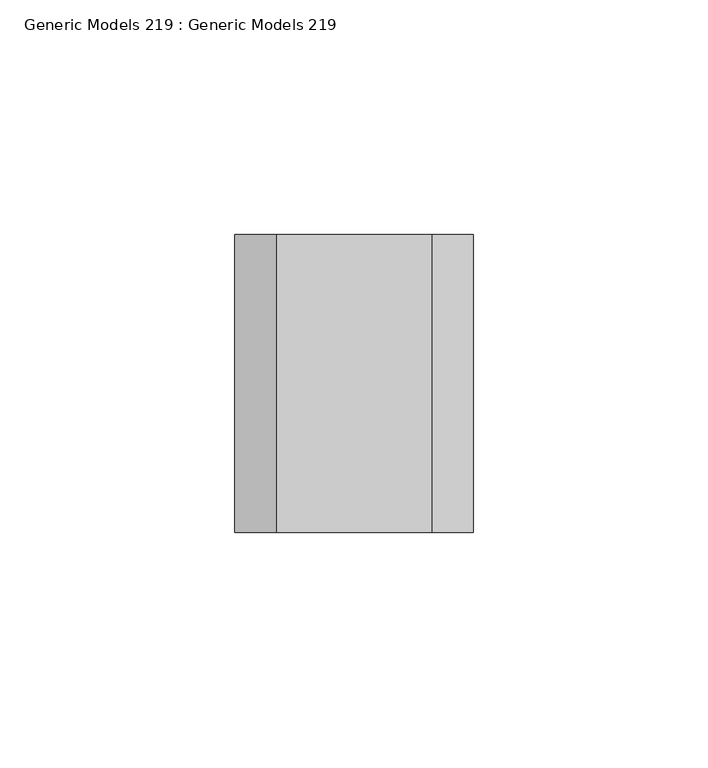
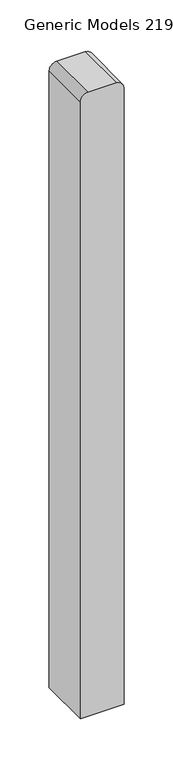
"""IFC4 building model written with IfcOpenShell, lengths in millimetres: proxy geometry, Generic Models 219 : Generic Models 219."""

import ifcopenshell
import ifcopenshell.guid

model = None  # the IFC model being written
_history = None  # IfcOwnerHistory: only IFC2X3 demands one
_inside = {}  # id of a spatial element -> (the spatial element, [elements in it])
_under = {}  # id of a project, library or spatial element -> (it, [spatial elements below it])
_declared = {}  # id of a project -> (the project, [libraries it declares])
_typed = {}  # id of a type object -> (the type object, [elements of that type])
_made_of = {}  # id of a material, layer set ... -> (it, [elements and type objects made of it])


def new_model(schema):
    """Start an empty IFC model of exactly this schema.

    Asked for "IFC4X3", IfcOpenShell would pick the latest addendum, in which some entities
    have other attributes; the version numbers below select the first issue.
    IFC2X3 requires an IfcOwnerHistory on every rooted entity: one is made here for all.
    """
    global model, _history
    if schema == "IFC4X3":
        model = ifcopenshell.file(schema_version=(4, 3, 0, 0))
    else:
        model = ifcopenshell.file(schema=schema)
    _inside.clear()
    _under.clear()
    _declared.clear()
    _typed.clear()
    _made_of.clear()
    _history = None
    if model.schema == "IFC2X3":
        org = make("IfcOrganization", Name="unknown")
        user = make(
            "IfcPersonAndOrganization",
            ThePerson=make("IfcPerson", FamilyName="unknown"),
            TheOrganization=org,
        )
        app = make(
            "IfcApplication",
            ApplicationDeveloper=org,
            Version="unknown",
            ApplicationFullName="unknown",
            ApplicationIdentifier="unknown",
        )
        _history = make(
            "IfcOwnerHistory",
            OwningUser=user,
            OwningApplication=app,
            ChangeAction="ADDED",
            CreationDate=0,
        )
    return model


def make(cls, **values):
    """One entity of the class cls with the attributes given. An attribute that is None is left unset."""
    return model.create_entity(
        cls, **{name: value for name, value in values.items() if value is not None}
    )


def rooted(cls, **values):
    """An entity with a GlobalId (a new one), such as an element, a storey or a relation."""
    return make(cls, GlobalId=ifcopenshell.guid.new(), OwnerHistory=_history, **values)


def si_unit(unit_type, name, prefix=None):
    """IfcSIUnit, for example si_unit("LENGTHUNIT", "METRE", prefix="MILLI")."""
    return make("IfcSIUnit", UnitType=unit_type, Prefix=prefix, Name=name)


def assignment(units):
    """IfcUnitAssignment: the units of a project."""
    return None if units is None else make("IfcUnitAssignment", Units=units)


def point(xyz):
    """IfcCartesianPoint."""
    return None if xyz is None else make("IfcCartesianPoint", Coordinates=xyz)


def direction(xyz):
    """IfcDirection."""
    return None if xyz is None else make("IfcDirection", DirectionRatios=xyz)


def frame(location, z_axis=None, x_axis=None):
    """IfcAxis2Placement3D, a coordinate frame: its origin and axes. An axis left out is left unset."""
    return make(
        "IfcAxis2Placement3D",
        Location=point(location),
        Axis=direction(z_axis),
        RefDirection=direction(x_axis),
    )


def frame_2d(location, x_axis=None):
    """IfcAxis2Placement2D, a coordinate frame in the plane: its origin and x axis."""
    return make(
        "IfcAxis2Placement2D", Location=point(location), RefDirection=direction(x_axis)
    )


def origin():
    """The frame at (0, 0, 0) with its axes left unset."""
    return frame((0.0, 0.0, 0.0))


def place(relative_to, where):
    """IfcLocalPlacement: puts the frame where relative to a parent placement (None: the world)."""
    return make(
        "IfcLocalPlacement", PlacementRelTo=relative_to, RelativePlacement=where
    )


def context(
    kind, dimensions, precision=None, world=None, true_north=None, identifier=None
):
    """IfcGeometricRepresentationContext, for example the 3D "Model" context."""
    return make(
        "IfcGeometricRepresentationContext",
        ContextIdentifier=identifier,
        ContextType=kind,
        CoordinateSpaceDimension=dimensions,
        Precision=precision,
        WorldCoordinateSystem=world,
        TrueNorth=true_north,
    )


def project(units=None, contexts=None):
    """IfcProject with its units and contexts."""
    return rooted(
        "IfcProject",
        Name="project",
        RepresentationContexts=contexts,
        UnitsInContext=assignment(units),
    )


def spatial(cls, under=None, at=None, **own):
    """A site, building, storey or space (cls), placed at a placement, below another one or the project."""
    s = rooted(cls, ObjectPlacement=at, **own)
    if under is not None:
        _under.setdefault(under.id(), (under, []))[1].append(s)
    return s


def polyline(points):
    """IfcPolyline through the points."""
    return make("IfcPolyline", Points=[point(p) for p in points])


def circle_curve(where, radius):
    """IfcCircle in the frame where."""
    return make("IfcCircle", Position=where, Radius=radius)


def trimmed(basis, trim1, trim2, sense, master):
    """IfcTrimmedCurve: the piece of a basis curve between two trims."""
    return make(
        "IfcTrimmedCurve",
        BasisCurve=basis,
        Trim1=trim1,
        Trim2=trim2,
        SenseAgreement=sense,
        MasterRepresentation=master,
    )


def segment(curve, same_sense, transition):
    """IfcCompositeCurveSegment."""
    return make(
        "IfcCompositeCurveSegment",
        Transition=transition,
        SameSense=same_sense,
        ParentCurve=curve,
    )


def composite_curve(segments, self_intersect=None):
    """IfcCompositeCurve: segments joined end to end."""
    return make("IfcCompositeCurve", Segments=segments, SelfIntersect=self_intersect)


def outline(outer, holes=None, kind="AREA"):
    """IfcArbitraryClosedProfileDef: a profile drawn as a closed curve; with holes, ...WithVoids."""
    if holes is None:
        return make("IfcArbitraryClosedProfileDef", ProfileType=kind, OuterCurve=outer)
    return make(
        "IfcArbitraryProfileDefWithVoids",
        ProfileType=kind,
        OuterCurve=outer,
        InnerCurves=holes,
    )


def extrude(swept, where, along, depth):
    """IfcExtrudedAreaSolid: the profile swept, set in the frame where, extruded along a direction by depth."""
    return make(
        "IfcExtrudedAreaSolid",
        SweptArea=swept,
        Position=where,
        ExtrudedDirection=direction(along),
        Depth=depth,
    )


def shape(context_of_items, identifier, shape_type, items):
    """IfcShapeRepresentation: the items that make up one representation, for example the "Body"."""
    return make(
        "IfcShapeRepresentation",
        ContextOfItems=context_of_items,
        RepresentationIdentifier=identifier,
        RepresentationType=shape_type,
        Items=items,
    )


def source(mapping_origin, context_of_items, identifier, shape_type, items):
    """IfcRepresentationMap: a shape defined once, which mapped items show again and again."""
    return make(
        "IfcRepresentationMap",
        MappingOrigin=mapping_origin,
        MappedRepresentation=shape(context_of_items, identifier, shape_type, items),
    )


def transform(
    local_origin,
    x_axis=None,
    y_axis=None,
    z_axis=None,
    scale=None,
    scale2=None,
    scale3=None,
    uniform=True,
):
    """IfcCartesianTransformationOperator3D, or its non-uniform kind. x_axis, y_axis, z_axis: its Axis1, 2, 3."""
    if uniform:
        return make(
            "IfcCartesianTransformationOperator3D",
            Axis1=direction(x_axis),
            Axis2=direction(y_axis),
            LocalOrigin=point(local_origin),
            Scale=scale,
            Axis3=direction(z_axis),
        )
    return make(
        "IfcCartesianTransformationOperator3DnonUniform",
        Axis1=direction(x_axis),
        Axis2=direction(y_axis),
        LocalOrigin=point(local_origin),
        Scale=scale,
        Axis3=direction(z_axis),
        Scale2=scale2,
        Scale3=scale3,
    )


def mapped(mapping_source, mapping_target):
    """IfcMappedItem: shows the shape of a source again, moved by a transform."""
    return make(
        "IfcMappedItem", MappingSource=mapping_source, MappingTarget=mapping_target
    )


def made_of(thing, what):
    """Note that an element or type object is made of a material, layer set ...; save() writes the relation."""
    if what is not None:
        _made_of.setdefault(what.id(), (what, []))[1].append(thing)
    return thing


def element(
    cls,
    number,
    at=None,
    inside=None,
    cuts=None,
    type_object=None,
    material=None,
    context=None,
    identifier="Body",
    shape_type=None,
    held_by="IfcProductDefinitionShape",
    body=None,
    shapes=None,
    **own,
):
    """One element of the class cls, such as IfcWall. Its Tag is "e" and its number.

    at: its placement. inside: the storey or other place that contains it. cuts: it is an
    opening in that element (IfcRelVoidsElement). A single representation is given by context,
    identifier, shape_type and body (its items); several are given by shapes. held_by: the class
    of the entity that holds the representations. save() writes the other relations.
    """
    e = rooted(cls, Tag="e%d" % number, ObjectPlacement=at, **own)
    if body is not None:
        shapes = [shape(context, identifier, shape_type, body)]
    if shapes is not None:
        e.Representation = make(held_by, Representations=shapes)
    if inside is not None:
        _inside.setdefault(inside.id(), (inside, []))[1].append(e)
    if cuts is not None:
        rooted(
            "IfcRelVoidsElement", RelatingBuildingElement=cuts, RelatedOpeningElement=e
        )
    if type_object is not None:
        _typed.setdefault(type_object.id(), (type_object, []))[1].append(e)
    return made_of(e, material)


def aggregate(whole, parts):
    """IfcRelAggregates: a whole, such as a stair, and the parts it consists of."""
    return rooted("IfcRelAggregates", RelatingObject=whole, RelatedObjects=parts)


def save(model, path):
    """Write the relations noted so far, then the file.

    IfcRelAggregates (storeys below a building ...), IfcRelContainedInSpatialStructure (elements
    in a storey), IfcRelDefinesByType, IfcRelAssociatesMaterial and IfcRelDeclares: one each for
    every whole, place, type object, material and project.
    """
    for whole, parts in _under.values():
        aggregate(whole, parts)
    for where, things in _inside.values():
        rooted(
            "IfcRelContainedInSpatialStructure",
            RelatedElements=things,
            RelatingStructure=where,
        )
    for kind, things in _typed.values():
        rooted("IfcRelDefinesByType", RelatedObjects=things, RelatingType=kind)
    for what, things in _made_of.values():
        rooted("IfcRelAssociatesMaterial", RelatedObjects=things, RelatingMaterial=what)
    for by, libraries in _declared.values():
        rooted("IfcRelDeclares", RelatingContext=by, RelatedDefinitions=libraries)
    model.write(path)


def generic_models_219_generic_models_219_1114332a(model_context):
    return source(origin(), model_context, "Body", "SweptSolid", [
        extrude(outline(composite_curve([segment(polyline([(126235.7571172, 7829.3763704), (125473.1746907, 7829.3763704), (125473.1746907, 7880.1763704), (126235.7571172, 7880.1763704)]), True, "CONTINUOUS"), segment(trimmed(circle_curve(frame_2d((126235.7571172, 7871.3371704)), 8.8392), [point((126235.7571172, 7880.1763704))], [point((126244.5963172, 7871.3371704))], False, "CARTESIAN"), True, "CONTINUOUS"), segment(polyline([(126244.5963172, 7871.3371704), (126244.5963172, 7838.2155704)]), True, "CONTINUOUS"), segment(trimmed(circle_curve(frame_2d((126235.7571172, 7838.2155704)), 8.8392), [point((126244.5963172, 7838.2155704))], [point((126235.7571172, 7829.3763704))], False, "CARTESIAN"), True, "CONTINUOUS")], self_intersect=False)), frame((0.0, 4501.3863946, 0.0), z_axis=(0.0, 1.0, 0.0), x_axis=(0.0, 0.0, 1.0)), (0.0, 0.0, 1.0), 63.500874),
    ])


if __name__ == "__main__":
    model = new_model("IFC4")
    model_context = context("Model", 3, world=origin())
    ifc_project = project(units=[si_unit("LENGTHUNIT", "METRE", prefix="MILLI")], contexts=[model_context])
    site = spatial("IfcSite", under=ifc_project)
    building = spatial("IfcBuilding", under=site)
    placement = place(None, origin())
    generic_models_219_generic_models_219_shape = generic_models_219_generic_models_219_1114332a(model_context)
    element("IfcBuildingElementProxy", 1, Name="Generic Models 219 : Generic Models 219", ObjectType="Generic Models 219 : Generic Models 219", at=placement, inside=building, context=model_context, shape_type="MappedRepresentation", body=[
        mapped(generic_models_219_generic_models_219_shape, transform((0.0, 0.0, 0.0), x_axis=(1.0, 0.0, 0.0), y_axis=(0.0, 1.0, 0.0), z_axis=(0.0, 0.0, 1.0))),
    ])
    save(model, "model.ifc")

# Revit data of these elements
# Element 1 (IfcBuildingElementProxy, "Generic Models 219 : Generic Models 219")
#   Materials on its faces: "_2x3 STEEL PROFILE - METALIZED, PRIMED & PAINTED (COLOR PER ARCHITECT)"
# Materials
#   "_2x3 STEEL PROFILE - METALIZED, PRIMED & PAINTED (COLOR PER ARCHITECT)": class "Metal", colour RGB 199 199 199, transparency 0, Description = "Structural steel 50ksi", Cost = 0
